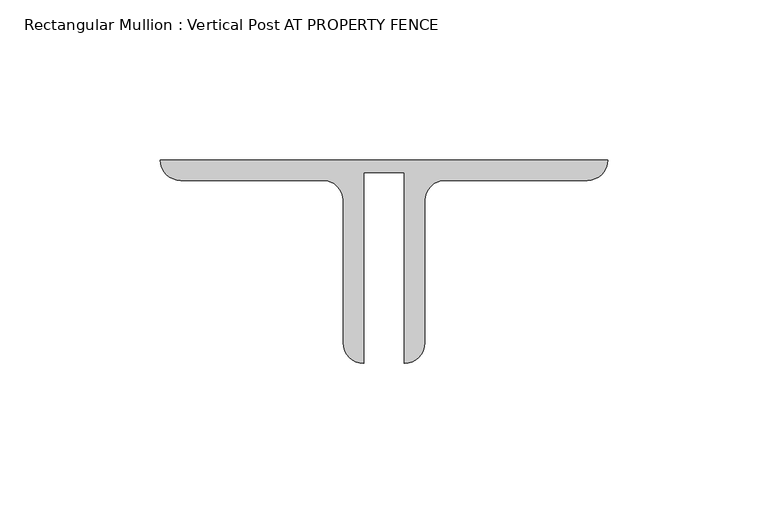
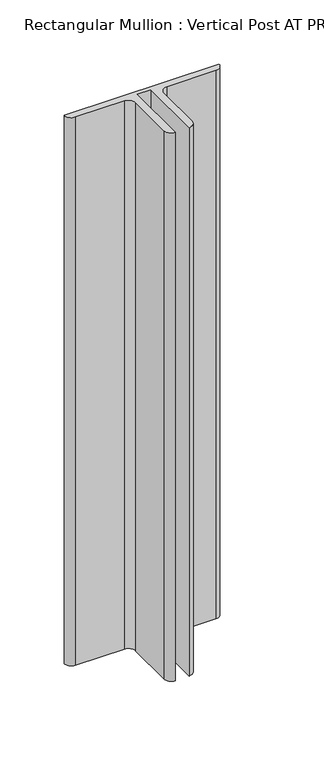
"""IFC4 building model written with IfcOpenShell, lengths in millimetres: member geometry, Rectangular Mullion : Vertical Post AT PROPERTY FENCE."""

from ifc_helpers import new_model, si_unit, point, frame, frame_2d, origin, place, context, project, spatial, polyline, circle_curve, trimmed, segment, composite_curve, outline, extrude, source, transform, mapped, element, save


def rectangular_mullion_vertical_post_at_property_fence_65e7824f(model_context):
    return source(origin(), model_context, "Body", "SweptSolid", [
        extrude(outline(composite_curve([segment(polyline([(-76.2, -22.9145205), (-76.2, -82.55)]), True, "CONTINUOUS"), segment(trimmed(circle_curve(frame_2d((-76.2, -76.2)), 6.35), [point((-76.2, -82.55))], [point((-82.55, -76.2))], False, "CARTESIAN"), True, "CONTINUOUS"), segment(polyline([(-82.55, -76.2), (-82.55, -31.75)]), True, "CONTINUOUS"), segment(trimmed(circle_curve(frame_2d((-88.9, -31.75)), 6.35), [point((-82.55, -31.75))], [point((-88.9, -25.4))], True, "CARTESIAN"), True, "CONTINUOUS"), segment(polyline([(-88.9, -25.4), (-133.35, -25.4)]), True, "CONTINUOUS"), segment(trimmed(circle_curve(frame_2d((-133.35, -19.05)), 6.35), [point((-133.35, -25.4))], [point((-139.7, -19.05))], False, "CARTESIAN"), True, "CONTINUOUS"), segment(polyline([(-139.7, -19.05), (0.0, -19.05)]), True, "CONTINUOUS"), segment(trimmed(circle_curve(frame_2d((-6.35, -19.05)), 6.35), [point((0.0, -19.05))], [point((-6.35, -25.4))], False, "CARTESIAN"), True, "CONTINUOUS"), segment(polyline([(-6.35, -25.4), (-50.8, -25.4)]), True, "CONTINUOUS"), segment(trimmed(circle_curve(frame_2d((-50.8, -31.75)), 6.35), [point((-50.8, -25.4))], [point((-57.15, -31.75))], True, "CARTESIAN"), True, "CONTINUOUS"), segment(polyline([(-57.15, -31.75), (-57.15, -76.2)]), True, "CONTINUOUS"), segment(trimmed(circle_curve(frame_2d((-63.5, -76.2)), 6.35), [point((-57.15, -76.2))], [point((-63.5, -82.55))], False, "CARTESIAN"), True, "CONTINUOUS"), segment(polyline([(-63.5, -82.55), (-63.5, -22.9145205), (-76.2, -22.9145205)]), True, "CONTINUOUS")], self_intersect=False)), frame((0.0, 0.0, -522.9663052), z_axis=(0.0, 0.0, 1.0), x_axis=(1.0, 0.0, 0.0)), (0.0, 0.0, 1.0), 522.9663052),
    ])


if __name__ == "__main__":
    model = new_model("IFC4")
    model_context = context("Model", 3, world=origin())
    ifc_project = project(units=[si_unit("LENGTHUNIT", "METRE", prefix="MILLI")], contexts=[model_context])
    site = spatial("IfcSite", under=ifc_project)
    building = spatial("IfcBuilding", under=site)
    placement = place(None, origin())
    rectangular_mullion_vertical_post_at_property_fence_shape = rectangular_mullion_vertical_post_at_property_fence_65e7824f(model_context)
    element("IfcMember", 1, ObjectType="Rectangular Mullion : Vertical Post AT PROPERTY FENCE", at=placement, inside=building, context=model_context, shape_type="MappedRepresentation", body=[
        mapped(rectangular_mullion_vertical_post_at_property_fence_shape, transform((0.0, 0.0, 0.0), x_axis=(1.0, 0.0, 0.0), y_axis=(0.0, 1.0, 0.0), z_axis=(0.0, 0.0, 1.0))),
    ])
    save(model, "model.ifc")

# Revit data of these elements
# Type "Rectangular Mullion : Vertical Post AT PROPERTY FENCE"
#   built-in parameter 1007351 = -0.0625 (stored number, unit not read)
#   built-in parameter 1007322 = 0.0126789 (stored number, unit not read)
#   built-in parameter 1007321 = 0.229167 (stored number, unit not read)
#   built-in parameter 1007320 = 0.229167 (stored number, unit not read)
# Element 1 (IfcMember, "Rectangular Mullion : Vertical Post AT PROPERTY FENCE")
#   Materials on its faces: "MAIN FENCE POST: (2) BACK/BACK GALVANIZED ANGLES (2) L2 1/2 X 2 1/2 X 1/4\") ANCHORED TO 8\"W X 42\" DEEP CONCRETE FOOTING(1)"
# Materials
#   "MAIN FENCE POST: (2) BACK/BACK GALVANIZED ANGLES (2) L2 1/2 X 2 1/2 X 1/4\") ANCHORED TO 8\"W X 42\" DEEP CONCRETE FOOTING(1)": class "Unassigned", colour RGB 211 211 211, transparency 0, Cost = 0
